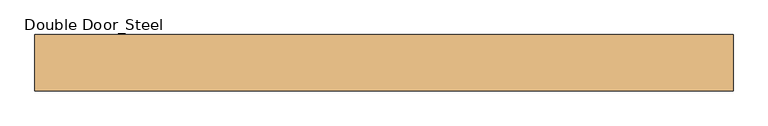
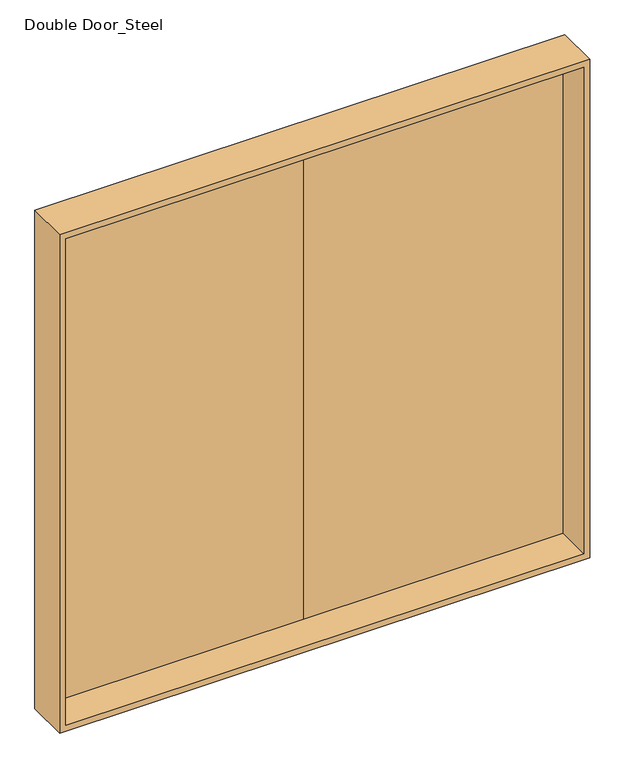
"""IFC4 building model written with IfcOpenShell, lengths in millimetres: door geometry, Double Door_Steel : H_DR_AR_B12_Double Door_Sliding_W3100xH3080_SD4."""

import ifcopenshell
import ifcopenshell.guid

model = None  # the IFC model being written
_history = None  # IfcOwnerHistory: only IFC2X3 demands one
_inside = {}  # id of a spatial element -> (the spatial element, [elements in it])
_under = {}  # id of a project, library or spatial element -> (it, [spatial elements below it])
_declared = {}  # id of a project -> (the project, [libraries it declares])
_typed = {}  # id of a type object -> (the type object, [elements of that type])
_made_of = {}  # id of a material, layer set ... -> (it, [elements and type objects made of it])


def new_model(schema):
    """Start an empty IFC model of exactly this schema.

    Asked for "IFC4X3", IfcOpenShell would pick the latest addendum, in which some entities
    have other attributes; the version numbers below select the first issue.
    IFC2X3 requires an IfcOwnerHistory on every rooted entity: one is made here for all.
    """
    global model, _history
    if schema == "IFC4X3":
        model = ifcopenshell.file(schema_version=(4, 3, 0, 0))
    else:
        model = ifcopenshell.file(schema=schema)
    _inside.clear()
    _under.clear()
    _declared.clear()
    _typed.clear()
    _made_of.clear()
    _history = None
    if model.schema == "IFC2X3":
        org = make("IfcOrganization", Name="unknown")
        user = make(
            "IfcPersonAndOrganization",
            ThePerson=make("IfcPerson", FamilyName="unknown"),
            TheOrganization=org,
        )
        app = make(
            "IfcApplication",
            ApplicationDeveloper=org,
            Version="unknown",
            ApplicationFullName="unknown",
            ApplicationIdentifier="unknown",
        )
        _history = make(
            "IfcOwnerHistory",
            OwningUser=user,
            OwningApplication=app,
            ChangeAction="ADDED",
            CreationDate=0,
        )
    return model


def make(cls, **values):
    """One entity of the class cls with the attributes given. An attribute that is None is left unset."""
    return model.create_entity(
        cls, **{name: value for name, value in values.items() if value is not None}
    )


def rooted(cls, **values):
    """An entity with a GlobalId (a new one), such as an element, a storey or a relation."""
    return make(cls, GlobalId=ifcopenshell.guid.new(), OwnerHistory=_history, **values)


def si_unit(unit_type, name, prefix=None):
    """IfcSIUnit, for example si_unit("LENGTHUNIT", "METRE", prefix="MILLI")."""
    return make("IfcSIUnit", UnitType=unit_type, Prefix=prefix, Name=name)


def assignment(units):
    """IfcUnitAssignment: the units of a project."""
    return None if units is None else make("IfcUnitAssignment", Units=units)


def point(xyz):
    """IfcCartesianPoint."""
    return None if xyz is None else make("IfcCartesianPoint", Coordinates=xyz)


def direction(xyz):
    """IfcDirection."""
    return None if xyz is None else make("IfcDirection", DirectionRatios=xyz)


def frame(location, z_axis=None, x_axis=None):
    """IfcAxis2Placement3D, a coordinate frame: its origin and axes. An axis left out is left unset."""
    return make(
        "IfcAxis2Placement3D",
        Location=point(location),
        Axis=direction(z_axis),
        RefDirection=direction(x_axis),
    )


def origin():
    """The frame at (0, 0, 0) with its axes left unset."""
    return frame((0.0, 0.0, 0.0))


def place(relative_to, where):
    """IfcLocalPlacement: puts the frame where relative to a parent placement (None: the world)."""
    return make(
        "IfcLocalPlacement", PlacementRelTo=relative_to, RelativePlacement=where
    )


def context(
    kind, dimensions, precision=None, world=None, true_north=None, identifier=None
):
    """IfcGeometricRepresentationContext, for example the 3D "Model" context."""
    return make(
        "IfcGeometricRepresentationContext",
        ContextIdentifier=identifier,
        ContextType=kind,
        CoordinateSpaceDimension=dimensions,
        Precision=precision,
        WorldCoordinateSystem=world,
        TrueNorth=true_north,
    )


def project(units=None, contexts=None):
    """IfcProject with its units and contexts."""
    return rooted(
        "IfcProject",
        Name="project",
        RepresentationContexts=contexts,
        UnitsInContext=assignment(units),
    )


def spatial(cls, under=None, at=None, **own):
    """A site, building, storey or space (cls), placed at a placement, below another one or the project."""
    s = rooted(cls, ObjectPlacement=at, **own)
    if under is not None:
        _under.setdefault(under.id(), (under, []))[1].append(s)
    return s


def polyline(points):
    """IfcPolyline through the points."""
    return make("IfcPolyline", Points=[point(p) for p in points])


def outline(outer, holes=None, kind="AREA"):
    """IfcArbitraryClosedProfileDef: a profile drawn as a closed curve; with holes, ...WithVoids."""
    if holes is None:
        return make("IfcArbitraryClosedProfileDef", ProfileType=kind, OuterCurve=outer)
    return make(
        "IfcArbitraryProfileDefWithVoids",
        ProfileType=kind,
        OuterCurve=outer,
        InnerCurves=holes,
    )


def extrude(swept, where, along, depth):
    """IfcExtrudedAreaSolid: the profile swept, set in the frame where, extruded along a direction by depth."""
    return make(
        "IfcExtrudedAreaSolid",
        SweptArea=swept,
        Position=where,
        ExtrudedDirection=direction(along),
        Depth=depth,
    )


def faces_of(points, faces, orient=None, outer=None):
    """IfcFace entities. A face is a list of loops; a loop is a list of indices into points, from 0.

    orient and outer hold one flag for each loop. By default every Orientation is true, the
    first loop of a face is its IfcFaceOuterBound and the others are IfcFaceBound.
    """
    made = []
    for i, loops in enumerate(faces):
        bounds = []
        for j, loop in enumerate(loops):
            is_outer = j == 0 if outer is None else outer[i][j]
            bounds.append(
                make(
                    "IfcFaceOuterBound" if is_outer else "IfcFaceBound",
                    Bound=make("IfcPolyLoop", Polygon=[points[k] for k in loop]),
                    Orientation=True if orient is None else orient[i][j],
                )
            )
        made.append(make("IfcFace", Bounds=bounds))
    return made


def faceted_brep(points, faces, orient=None, outer=None, voids=None):
    """IfcFacetedBrep: a solid bounded by flat faces; with voids (closed shells), ...WithVoids."""
    shared = [point(p) for p in points]
    hull = make("IfcClosedShell", CfsFaces=faces_of(shared, faces, orient, outer))
    if voids is None:
        return make("IfcFacetedBrep", Outer=hull)
    return make(
        "IfcFacetedBrepWithVoids",
        Outer=hull,
        Voids=[
            make(cls, CfsFaces=faces_of(shared, fs, o, b)) for cls, fs, o, b in voids
        ],
    )


def shape(context_of_items, identifier, shape_type, items):
    """IfcShapeRepresentation: the items that make up one representation, for example the "Body"."""
    return make(
        "IfcShapeRepresentation",
        ContextOfItems=context_of_items,
        RepresentationIdentifier=identifier,
        RepresentationType=shape_type,
        Items=items,
    )


def source(mapping_origin, context_of_items, identifier, shape_type, items):
    """IfcRepresentationMap: a shape defined once, which mapped items show again and again."""
    return make(
        "IfcRepresentationMap",
        MappingOrigin=mapping_origin,
        MappedRepresentation=shape(context_of_items, identifier, shape_type, items),
    )


def transform(
    local_origin,
    x_axis=None,
    y_axis=None,
    z_axis=None,
    scale=None,
    scale2=None,
    scale3=None,
    uniform=True,
):
    """IfcCartesianTransformationOperator3D, or its non-uniform kind. x_axis, y_axis, z_axis: its Axis1, 2, 3."""
    if uniform:
        return make(
            "IfcCartesianTransformationOperator3D",
            Axis1=direction(x_axis),
            Axis2=direction(y_axis),
            LocalOrigin=point(local_origin),
            Scale=scale,
            Axis3=direction(z_axis),
        )
    return make(
        "IfcCartesianTransformationOperator3DnonUniform",
        Axis1=direction(x_axis),
        Axis2=direction(y_axis),
        LocalOrigin=point(local_origin),
        Scale=scale,
        Axis3=direction(z_axis),
        Scale2=scale2,
        Scale3=scale3,
    )


def mapped(mapping_source, mapping_target):
    """IfcMappedItem: shows the shape of a source again, moved by a transform."""
    return make(
        "IfcMappedItem", MappingSource=mapping_source, MappingTarget=mapping_target
    )


def made_of(thing, what):
    """Note that an element or type object is made of a material, layer set ...; save() writes the relation."""
    if what is not None:
        _made_of.setdefault(what.id(), (what, []))[1].append(thing)
    return thing


def element(
    cls,
    number,
    at=None,
    inside=None,
    cuts=None,
    type_object=None,
    material=None,
    context=None,
    identifier="Body",
    shape_type=None,
    held_by="IfcProductDefinitionShape",
    body=None,
    shapes=None,
    **own,
):
    """One element of the class cls, such as IfcWall. Its Tag is "e" and its number.

    at: its placement. inside: the storey or other place that contains it. cuts: it is an
    opening in that element (IfcRelVoidsElement). A single representation is given by context,
    identifier, shape_type and body (its items); several are given by shapes. held_by: the class
    of the entity that holds the representations. save() writes the other relations.
    """
    e = rooted(cls, Tag="e%d" % number, ObjectPlacement=at, **own)
    if body is not None:
        shapes = [shape(context, identifier, shape_type, body)]
    if shapes is not None:
        e.Representation = make(held_by, Representations=shapes)
    if inside is not None:
        _inside.setdefault(inside.id(), (inside, []))[1].append(e)
    if cuts is not None:
        rooted(
            "IfcRelVoidsElement", RelatingBuildingElement=cuts, RelatedOpeningElement=e
        )
    if type_object is not None:
        _typed.setdefault(type_object.id(), (type_object, []))[1].append(e)
    return made_of(e, material)


def aggregate(whole, parts):
    """IfcRelAggregates: a whole, such as a stair, and the parts it consists of."""
    return rooted("IfcRelAggregates", RelatingObject=whole, RelatedObjects=parts)


def save(model, path):
    """Write the relations noted so far, then the file.

    IfcRelAggregates (storeys below a building ...), IfcRelContainedInSpatialStructure (elements
    in a storey), IfcRelDefinesByType, IfcRelAssociatesMaterial and IfcRelDeclares: one each for
    every whole, place, type object, material and project.
    """
    for whole, parts in _under.values():
        aggregate(whole, parts)
    for where, things in _inside.values():
        rooted(
            "IfcRelContainedInSpatialStructure",
            RelatedElements=things,
            RelatingStructure=where,
        )
    for kind, things in _typed.values():
        rooted("IfcRelDefinesByType", RelatedObjects=things, RelatingType=kind)
    for what, things in _made_of.values():
        rooted("IfcRelAssociatesMaterial", RelatedObjects=things, RelatingMaterial=what)
    for by, libraries in _declared.values():
        rooted("IfcRelDeclares", RelatingContext=by, RelatedDefinitions=libraries)
    model.write(path)


def double_door_steel_99e35c84(model_context):
    return source(origin(), model_context, "Body", "SolidModel", [
        extrude(outline(polyline([(1530.0, 85.0), (0.0, 85.0), (0.0, 125.0), (1530.0, 125.0), (1530.0, 85.0)])), frame((0.0, 0.0, 20.0), z_axis=(0.0, 0.0, 1.0), x_axis=(1.0, 0.0, 0.0)), (0.0, 0.0, 1.0), 3040.0),
        extrude(outline(polyline([(0.0, 85.0), (-1530.0, 85.0), (-1530.0, 125.0), (0.0, 125.0), (0.0, 85.0)])), frame((0.0, 0.0, 20.0), z_axis=(0.0, 0.0, 1.0), x_axis=(1.0, 0.0, 0.0)), (0.0, 0.0, 1.0), 3040.0),
        faceted_brep([(1550.0, -125.0, 3080.0), (1550.0, 125.0, 3080.0), (-1550.0, 125.0, 3080.0), (-1550.0, -125.0, 3080.0), (1515.0, 85.0, 3045.0), (1515.0, -125.0, 3045.0), (-1515.0, -125.0, 3045.0), (-1515.0, 85.0, 3045.0), (1530.0, 125.0, 3060.0), (1530.0, 85.0, 3060.0), (-1530.0, 85.0, 3060.0), (-1530.0, 125.0, 3060.0), (-1550.0, 125.0, 0.0), (-1550.0, -125.0, 0.0), (-1515.0, -125.0, 35.0), (-1515.0, 85.0, 35.0), (-1530.0, 85.0, 20.0), (-1530.0, 125.0, 20.0), (1550.0, 125.0, 0.0), (1530.0, 125.0, 20.0), (1550.0, -125.0, 0.0), (1515.0, -125.0, 35.0), (1515.0, 85.0, 35.0), (1530.0, 85.0, 20.0)], [[[0, 1, 2, 3]], [[4, 5, 6, 7]], [[8, 9, 10, 11]], [[3, 2, 12, 13]], [[7, 6, 14, 15]], [[11, 10, 16, 17]], [[18, 12, 2, 1], [8, 11, 17, 19]], [[13, 12, 18, 20]], [[0, 3, 13, 20], [21, 14, 6, 5]], [[15, 14, 21, 22]], [[23, 16, 10, 9], [4, 7, 15, 22]], [[17, 16, 23, 19]], [[20, 18, 1, 0]], [[22, 21, 5, 4]], [[19, 23, 9, 8]]]),
    ])


if __name__ == "__main__":
    model = new_model("IFC4")
    model_context = context("Model", 3, world=origin())
    ifc_project = project(units=[si_unit("LENGTHUNIT", "METRE", prefix="MILLI")], contexts=[model_context])
    site = spatial("IfcSite", under=ifc_project)
    building = spatial("IfcBuilding", under=site)
    placement = place(None, origin())
    double_door_steel_shape = double_door_steel_99e35c84(model_context)
    element("IfcDoor", 1, ObjectType="Double Door_Steel : H_DR_AR_B12_Double Door_Sliding_W3100xH3080_SD4", at=placement, inside=building, context=model_context, shape_type="MappedRepresentation", body=[
        mapped(double_door_steel_shape, transform((0.0, 0.0, 0.0), x_axis=(1.0, 0.0, 0.0), y_axis=(0.0, 1.0, 0.0), z_axis=(0.0, 0.0, 1.0))),
    ])
    save(model, "model.ifc")

# Revit data of these elements
# Type "Double Door_Steel : H_DR_AR_B12_Double Door_Sliding_W3100xH3080_SD4"
#   Type Mark = "446"
#   프레임 = ""
#   철물 = ""
#   유리/마감 = ""
#   위치/개소 = ""
#   부호 = "1/SD"
#   문번호 = "4"
#   문기호 = "SD"
#   Analytic Construction = "<None>"
#   Height = 3080 mm
#   Width = 3100 mm
#   Define Thermal Properties by = 1
#   문 틀 = none
#   문 = none
#   Function = (empty or 0)
#   Assembly Code = ""
#   Wall Closure = (empty or 0)
